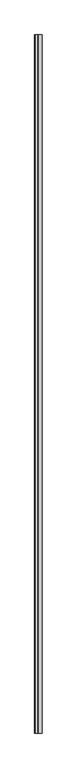
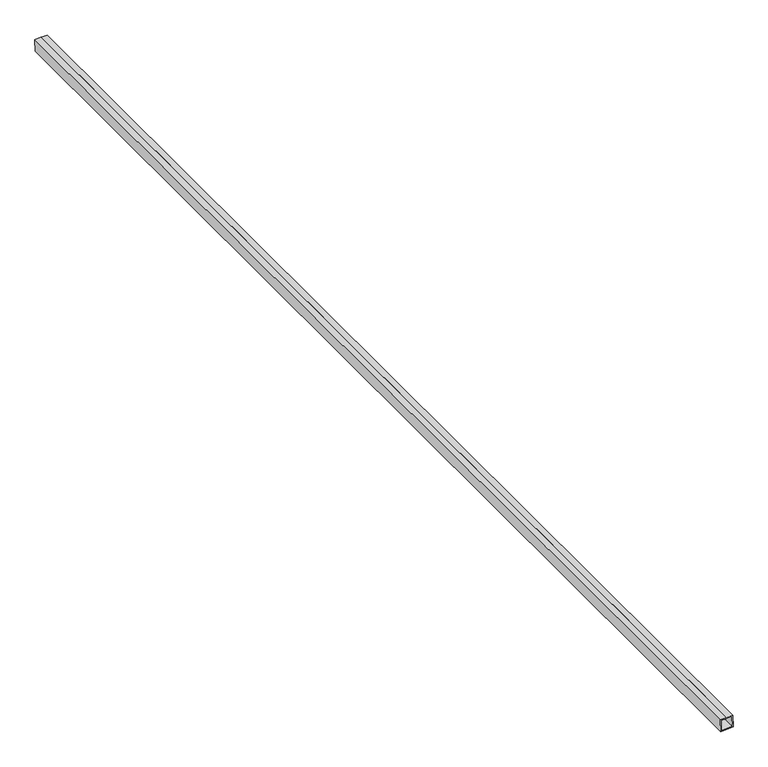
"""IFC4 building model written with IfcOpenShell, lengths in millimetres: proxy geometry, Inner panel:Inner panel:1:Inner panel:1 : Inner panel:Inner panel:300324:2:Inner panel:1:Inner panel:1 : Inner panel:Inner panel:300324:2 : Inner panel:Inner panel:1:Inner panel:1 : Inner panel:Inner panel:300324:300043:33 : Inner panel:Inner panel:1:Inner panel:1 : Inner panel:Inner panel:300324:2:Inner panel:1:Inner panel:1 : Inner panel:Inner panel:300324:2 : Inner panel:Inner panel:1:Inner panel:1 : Inner panel:Inner panel:300324:300043:308120."""

from ifc_helpers import new_model, si_unit, frame, origin, place, context, project, spatial, polyline, outline, extrude, source, transform, mapped, element, save


def generic_models_a9e2b546(model_context):
    return source(origin(), model_context, "Body", "SweptSolid", [
        extrude(outline(polyline([(4022.4868814, 562107.7864431), (4020.1076958, 562107.8855758), (4020.7685807, 562123.7468134), (3987.4599819, 562125.1346716), (3986.0721236, 562091.8260728), (4019.3807224, 562090.4382145), (4020.0416073, 562106.2994521), (4022.420793, 562106.2003193), (4021.6607753, 562087.9598962), (3983.5938052, 562089.5460199), (3985.179929, 562127.61299), (4023.2468991, 562126.0268663), (4022.4868814, 562107.7864431)])), frame((0.0, -579334.066384, 0.0), z_axis=(0.0, 1.0, 0.0), x_axis=(0.0, 0.0, 1.0)), (0.0, 0.0, 1.0), 3657.6),
    ])


if __name__ == "__main__":
    model = new_model("IFC4")
    model_context = context("Model", 3, world=origin())
    ifc_project = project(units=[si_unit("LENGTHUNIT", "METRE", prefix="MILLI")], contexts=[model_context])
    site = spatial("IfcSite", under=ifc_project)
    building = spatial("IfcBuilding", under=site)
    placement = place(None, origin())
    generic_models_shape = generic_models_a9e2b546(model_context)
    element("IfcBuildingElementProxy", 1, Name="Inner panel:Inner panel:1:Inner panel:1 : Inner panel:Inner panel:300324:2:Inner panel:1:Inner panel:1 : Inner panel:Inner panel:300324:2 : Inner panel:Inner panel:1:Inner panel:1 : Inner panel:Inner panel:300324:300043:33 : Inner panel:Inner panel:1:Inner panel:1 : Inner panel:Inner panel:300324:2:Inner panel:1:Inner panel:1 : Inner panel:Inner panel:300324:2 : Inner panel:Inner panel:1:Inner panel:1 : Inner panel:Inner panel:300324:300043:308120", ObjectType="Inner panel:Inner panel:1:Inner panel:1 : Inner panel:Inner panel:300324:2:Inner panel:1:Inner panel:1 : Inner panel:Inner panel:300324:2 : Inner panel:Inner panel:1:Inner panel:1 : Inner panel:Inner panel:300324:300043:33 : Inner panel:Inner panel:1:Inner panel:1 : Inner panel:Inner panel:300324:2:Inner panel:1:Inner panel:1 : Inner panel:Inner panel:300324:2 : Inner panel:Inner panel:1:Inner panel:1 : Inner panel:Inner panel:300324:300043:308120", at=placement, inside=building, context=model_context, shape_type="MappedRepresentation", body=[
        mapped(generic_models_shape, transform((0.0, 0.0, 0.0), x_axis=(1.0, 0.0, 0.0), y_axis=(0.0, 1.0, 0.0), z_axis=(0.0, 0.0, 1.0))),
    ])
    save(model, "model.ifc")

# Revit data of these elements
# Type "Inner panel:Inner panel:1:Inner panel:1 : Inner panel:Inner panel:300324:2:Inner panel:1:Inner panel:1 : Inner panel:Inner panel:300324:2 : Inner panel:Inner panel:1:Inner panel:1 : Inner panel:Inner panel:300324:300043:33 : Inner panel:Inner panel:1:Inner panel:1 : Inner panel:Inner panel:300324:2:Inner panel:1:Inner panel:1 : Inner panel:Inner panel:300324:2 : Inner panel:Inner panel:1:Inner panel:1 : Inner panel:Inner panel:300324:300043:308120"
#   NameOverride = "Inner panel:Inner panel:1:Inner panel:1 : Inner panel:Inner panel:300324:2:Inner panel:1:Inner panel:1 : Inner panel:Inner panel:300324:2 : Inner panel:Inner panel:1:Inner panel:1 : Inner panel:Inner panel:300324:300043:308120"
#   ObjectTypeOverride = "Inner panel:1:Inner panel:1 : Inner panel:Inner panel:300324:2 : Inner panel:Inner panel:1:Inner panel:1 : Inner panel:Inner panel:300324:300043"
#   Reference = "Inner panel"
#   Tag = "308120"
# Element 1 (IfcBuildingElementProxy, "Inner panel:Inner panel:1:Inner panel:1 : Inner panel:Inner panel:300324:2:Inner panel:1:Inner panel:1 : Inner panel:Inner panel:300324:2 : Inner panel:Inner panel:1:Inner panel:1 : Inner panel:Inner panel:300324:300043:33 : Inner panel:Inner panel:1:Inner panel:1 : Inner panel:Inner panel:300324:2:Inner panel:1:Inner panel:1 : Inner panel:Inner panel:300324:2 : Inner panel:Inner panel:1:Inner panel:1 : Inner panel:Inner panel:300324:300043:308120")
#   Materials on its faces: "1 1/2\" X 1 1/2\" SPLIT-SEAM SQUARE TUBING (~24\" CANTILEVER FROM C.L. OF GLULAM)"
# Materials
#   "1 1/2\" X 1 1/2\" SPLIT-SEAM SQUARE TUBING (~24\" CANTILEVER FROM C.L. OF GLULAM)": class "Unassigned", colour RGB 202 201 200, transparency 0, Cost = 0
